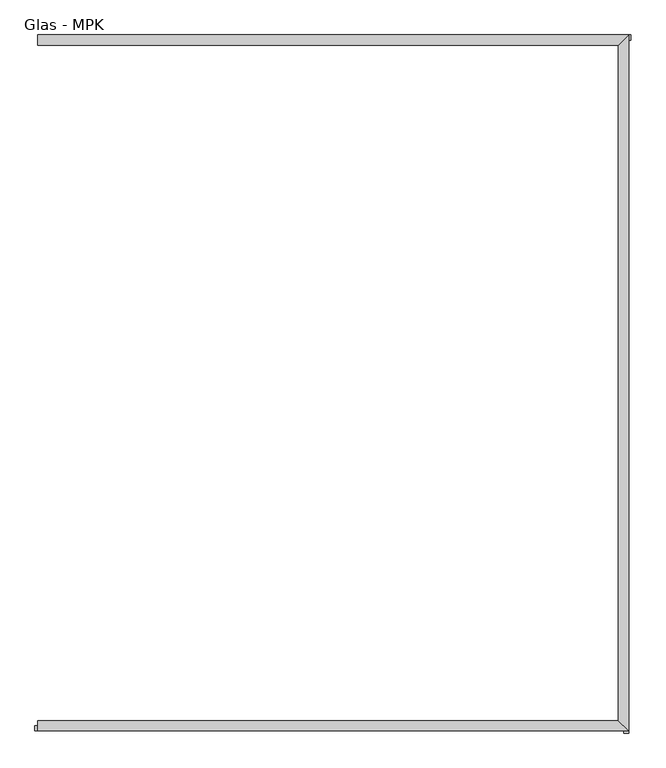
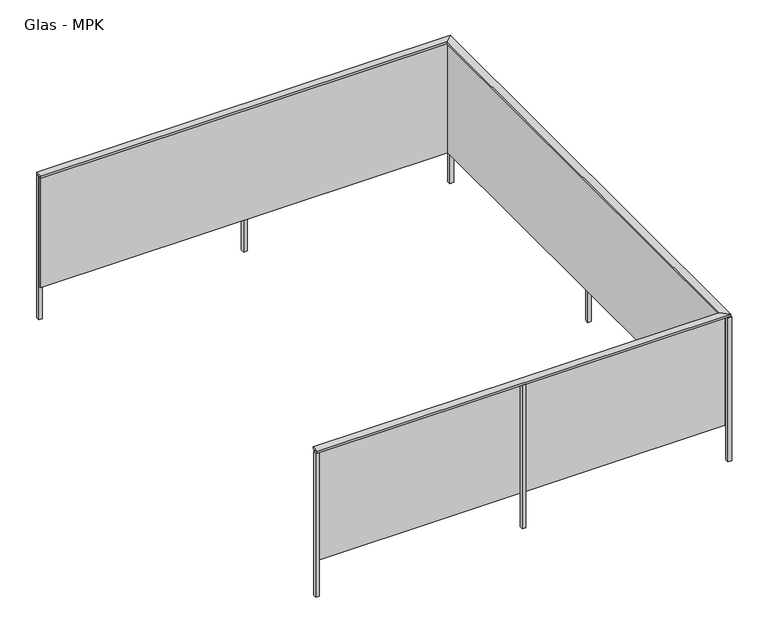
"""IFC4 building model written with IfcOpenShell, lengths in millimetres: railing geometry, Glas - MPK."""

import ifcopenshell
import ifcopenshell.guid

model = None  # the IFC model being written
_history = None  # IfcOwnerHistory: only IFC2X3 demands one
_inside = {}  # id of a spatial element -> (the spatial element, [elements in it])
_under = {}  # id of a project, library or spatial element -> (it, [spatial elements below it])
_declared = {}  # id of a project -> (the project, [libraries it declares])
_typed = {}  # id of a type object -> (the type object, [elements of that type])
_made_of = {}  # id of a material, layer set ... -> (it, [elements and type objects made of it])


def new_model(schema):
    """Start an empty IFC model of exactly this schema.

    Asked for "IFC4X3", IfcOpenShell would pick the latest addendum, in which some entities
    have other attributes; the version numbers below select the first issue.
    IFC2X3 requires an IfcOwnerHistory on every rooted entity: one is made here for all.
    """
    global model, _history
    if schema == "IFC4X3":
        model = ifcopenshell.file(schema_version=(4, 3, 0, 0))
    else:
        model = ifcopenshell.file(schema=schema)
    _inside.clear()
    _under.clear()
    _declared.clear()
    _typed.clear()
    _made_of.clear()
    _history = None
    if model.schema == "IFC2X3":
        org = make("IfcOrganization", Name="unknown")
        user = make(
            "IfcPersonAndOrganization",
            ThePerson=make("IfcPerson", FamilyName="unknown"),
            TheOrganization=org,
        )
        app = make(
            "IfcApplication",
            ApplicationDeveloper=org,
            Version="unknown",
            ApplicationFullName="unknown",
            ApplicationIdentifier="unknown",
        )
        _history = make(
            "IfcOwnerHistory",
            OwningUser=user,
            OwningApplication=app,
            ChangeAction="ADDED",
            CreationDate=0,
        )
    return model


def make(cls, **values):
    """One entity of the class cls with the attributes given. An attribute that is None is left unset."""
    return model.create_entity(
        cls, **{name: value for name, value in values.items() if value is not None}
    )


def rooted(cls, **values):
    """An entity with a GlobalId (a new one), such as an element, a storey or a relation."""
    return make(cls, GlobalId=ifcopenshell.guid.new(), OwnerHistory=_history, **values)


def si_unit(unit_type, name, prefix=None):
    """IfcSIUnit, for example si_unit("LENGTHUNIT", "METRE", prefix="MILLI")."""
    return make("IfcSIUnit", UnitType=unit_type, Prefix=prefix, Name=name)


def assignment(units):
    """IfcUnitAssignment: the units of a project."""
    return None if units is None else make("IfcUnitAssignment", Units=units)


def point(xyz):
    """IfcCartesianPoint."""
    return None if xyz is None else make("IfcCartesianPoint", Coordinates=xyz)


def direction(xyz):
    """IfcDirection."""
    return None if xyz is None else make("IfcDirection", DirectionRatios=xyz)


def frame(location, z_axis=None, x_axis=None):
    """IfcAxis2Placement3D, a coordinate frame: its origin and axes. An axis left out is left unset."""
    return make(
        "IfcAxis2Placement3D",
        Location=point(location),
        Axis=direction(z_axis),
        RefDirection=direction(x_axis),
    )


def origin():
    """The frame at (0, 0, 0) with its axes left unset."""
    return frame((0.0, 0.0, 0.0))


def place(relative_to, where):
    """IfcLocalPlacement: puts the frame where relative to a parent placement (None: the world)."""
    return make(
        "IfcLocalPlacement", PlacementRelTo=relative_to, RelativePlacement=where
    )


def context(
    kind, dimensions, precision=None, world=None, true_north=None, identifier=None
):
    """IfcGeometricRepresentationContext, for example the 3D "Model" context."""
    return make(
        "IfcGeometricRepresentationContext",
        ContextIdentifier=identifier,
        ContextType=kind,
        CoordinateSpaceDimension=dimensions,
        Precision=precision,
        WorldCoordinateSystem=world,
        TrueNorth=true_north,
    )


def project(units=None, contexts=None):
    """IfcProject with its units and contexts."""
    return rooted(
        "IfcProject",
        Name="project",
        RepresentationContexts=contexts,
        UnitsInContext=assignment(units),
    )


def spatial(cls, under=None, at=None, **own):
    """A site, building, storey or space (cls), placed at a placement, below another one or the project."""
    s = rooted(cls, ObjectPlacement=at, **own)
    if under is not None:
        _under.setdefault(under.id(), (under, []))[1].append(s)
    return s


def polyline(points):
    """IfcPolyline through the points."""
    return make("IfcPolyline", Points=[point(p) for p in points])


def outline(outer, holes=None, kind="AREA"):
    """IfcArbitraryClosedProfileDef: a profile drawn as a closed curve; with holes, ...WithVoids."""
    if holes is None:
        return make("IfcArbitraryClosedProfileDef", ProfileType=kind, OuterCurve=outer)
    return make(
        "IfcArbitraryProfileDefWithVoids",
        ProfileType=kind,
        OuterCurve=outer,
        InnerCurves=holes,
    )


def extrude(swept, where, along, depth):
    """IfcExtrudedAreaSolid: the profile swept, set in the frame where, extruded along a direction by depth."""
    return make(
        "IfcExtrudedAreaSolid",
        SweptArea=swept,
        Position=where,
        ExtrudedDirection=direction(along),
        Depth=depth,
    )


def faces_of(points, faces, orient=None, outer=None):
    """IfcFace entities. A face is a list of loops; a loop is a list of indices into points, from 0.

    orient and outer hold one flag for each loop. By default every Orientation is true, the
    first loop of a face is its IfcFaceOuterBound and the others are IfcFaceBound.
    """
    made = []
    for i, loops in enumerate(faces):
        bounds = []
        for j, loop in enumerate(loops):
            is_outer = j == 0 if outer is None else outer[i][j]
            bounds.append(
                make(
                    "IfcFaceOuterBound" if is_outer else "IfcFaceBound",
                    Bound=make("IfcPolyLoop", Polygon=[points[k] for k in loop]),
                    Orientation=True if orient is None else orient[i][j],
                )
            )
        made.append(make("IfcFace", Bounds=bounds))
    return made


def faceted_brep(points, faces, orient=None, outer=None, voids=None):
    """IfcFacetedBrep: a solid bounded by flat faces; with voids (closed shells), ...WithVoids."""
    shared = [point(p) for p in points]
    hull = make("IfcClosedShell", CfsFaces=faces_of(shared, faces, orient, outer))
    if voids is None:
        return make("IfcFacetedBrep", Outer=hull)
    return make(
        "IfcFacetedBrepWithVoids",
        Outer=hull,
        Voids=[
            make(cls, CfsFaces=faces_of(shared, fs, o, b)) for cls, fs, o, b in voids
        ],
    )


def shape(context_of_items, identifier, shape_type, items):
    """IfcShapeRepresentation: the items that make up one representation, for example the "Body"."""
    return make(
        "IfcShapeRepresentation",
        ContextOfItems=context_of_items,
        RepresentationIdentifier=identifier,
        RepresentationType=shape_type,
        Items=items,
    )


def source(mapping_origin, context_of_items, identifier, shape_type, items):
    """IfcRepresentationMap: a shape defined once, which mapped items show again and again."""
    return make(
        "IfcRepresentationMap",
        MappingOrigin=mapping_origin,
        MappedRepresentation=shape(context_of_items, identifier, shape_type, items),
    )


def transform(
    local_origin,
    x_axis=None,
    y_axis=None,
    z_axis=None,
    scale=None,
    scale2=None,
    scale3=None,
    uniform=True,
):
    """IfcCartesianTransformationOperator3D, or its non-uniform kind. x_axis, y_axis, z_axis: its Axis1, 2, 3."""
    if uniform:
        return make(
            "IfcCartesianTransformationOperator3D",
            Axis1=direction(x_axis),
            Axis2=direction(y_axis),
            LocalOrigin=point(local_origin),
            Scale=scale,
            Axis3=direction(z_axis),
        )
    return make(
        "IfcCartesianTransformationOperator3DnonUniform",
        Axis1=direction(x_axis),
        Axis2=direction(y_axis),
        LocalOrigin=point(local_origin),
        Scale=scale,
        Axis3=direction(z_axis),
        Scale2=scale2,
        Scale3=scale3,
    )


def mapped(mapping_source, mapping_target):
    """IfcMappedItem: shows the shape of a source again, moved by a transform."""
    return make(
        "IfcMappedItem", MappingSource=mapping_source, MappingTarget=mapping_target
    )


def made_of(thing, what):
    """Note that an element or type object is made of a material, layer set ...; save() writes the relation."""
    if what is not None:
        _made_of.setdefault(what.id(), (what, []))[1].append(thing)
    return thing


def element(
    cls,
    number,
    at=None,
    inside=None,
    cuts=None,
    type_object=None,
    material=None,
    context=None,
    identifier="Body",
    shape_type=None,
    held_by="IfcProductDefinitionShape",
    body=None,
    shapes=None,
    **own,
):
    """One element of the class cls, such as IfcWall. Its Tag is "e" and its number.

    at: its placement. inside: the storey or other place that contains it. cuts: it is an
    opening in that element (IfcRelVoidsElement). A single representation is given by context,
    identifier, shape_type and body (its items); several are given by shapes. held_by: the class
    of the entity that holds the representations. save() writes the other relations.
    """
    e = rooted(cls, Tag="e%d" % number, ObjectPlacement=at, **own)
    if body is not None:
        shapes = [shape(context, identifier, shape_type, body)]
    if shapes is not None:
        e.Representation = make(held_by, Representations=shapes)
    if inside is not None:
        _inside.setdefault(inside.id(), (inside, []))[1].append(e)
    if cuts is not None:
        rooted(
            "IfcRelVoidsElement", RelatingBuildingElement=cuts, RelatedOpeningElement=e
        )
    if type_object is not None:
        _typed.setdefault(type_object.id(), (type_object, []))[1].append(e)
    return made_of(e, material)


def aggregate(whole, parts):
    """IfcRelAggregates: a whole, such as a stair, and the parts it consists of."""
    return rooted("IfcRelAggregates", RelatingObject=whole, RelatedObjects=parts)


def save(model, path):
    """Write the relations noted so far, then the file.

    IfcRelAggregates (storeys below a building ...), IfcRelContainedInSpatialStructure (elements
    in a storey), IfcRelDefinesByType, IfcRelAssociatesMaterial and IfcRelDeclares: one each for
    every whole, place, type object, material and project.
    """
    for whole, parts in _under.values():
        aggregate(whole, parts)
    for where, things in _inside.values():
        rooted(
            "IfcRelContainedInSpatialStructure",
            RelatedElements=things,
            RelatingStructure=where,
        )
    for kind, things in _typed.values():
        rooted("IfcRelDefinesByType", RelatedObjects=things, RelatingType=kind)
    for what, things in _made_of.values():
        rooted("IfcRelAssociatesMaterial", RelatedObjects=things, RelatingMaterial=what)
    for by, libraries in _declared.values():
        rooted("IfcRelDeclares", RelatingContext=by, RelatedDefinitions=libraries)
    model.write(path)


def glas_mpk_050cb379(model_context):
    return source(origin(), model_context, "Body", "SolidModel", [
        faceted_brep([(28820.3199184, 1288.5335867, 3843.2628643), (28820.3199184, 1238.5335867, 3843.2628643), (28820.3199184, 1238.5335867, 3856.7371357), (28820.3199184, 1288.5335867, 3856.7371357), (31660.3199184, 1288.5335867, 3843.2628643), (31610.3199184, 1238.5335867, 3843.2628643), (31610.3199184, 1238.5335867, 3856.7371357), (31660.3199184, 1288.5335867, 3856.7371357), (31660.3199184, -2052.1957594, 3843.2628643), (31610.3199184, -2002.1957594, 3843.2628643), (31610.3199184, -2002.1957594, 3856.7371357), (31660.3199184, -2052.1957594, 3856.7371357), (28820.3199184, -2052.1957594, 3843.2628643), (28820.3199184, -2052.1957594, 3856.7371357), (28820.3199184, -2002.1957594, 3856.7371357), (28820.3199184, -2002.1957594, 3843.2628643)], [[[0, 1, 2, 3]], [[1, 0, 4, 5]], [[2, 1, 5, 6]], [[3, 2, 6, 7]], [[0, 3, 7, 4]], [[5, 4, 8, 9]], [[6, 5, 9, 10]], [[7, 6, 10, 11]], [[4, 7, 11, 8]], [[12, 13, 14, 15]], [[9, 8, 12, 15]], [[10, 9, 15, 14]], [[11, 10, 14, 13]], [[8, 11, 13, 12]]]),
        faceted_brep([(28820.3199184, 1248.5335867, 3842.8769824), (28820.3199184, 1262.7257107, 3842.8769824), (28820.3199184, 1262.7257107, 3042.8769824), (28820.3199184, 1248.5335867, 3042.8769824), (31620.3199184, 1248.5335867, 3842.8769824), (31634.5120424, 1262.7257107, 3842.8769824), (31634.5120424, 1262.7257107, 3042.8769824), (31620.3199184, 1248.5335867, 3042.8769824), (31620.3199184, -2012.1957594, 3842.8769824), (31634.5120424, -2026.3878834, 3842.8769824), (31634.5120424, -2026.3878834, 3042.8769824), (31620.3199184, -2012.1957594, 3042.8769824), (28820.3199184, -2012.1957594, 3842.8769824), (28820.3199184, -2012.1957594, 3042.8769824), (28820.3199184, -2026.3878834, 3042.8769824), (28820.3199184, -2026.3878834, 3842.8769824)], [[[0, 1, 2, 3]], [[1, 0, 4, 5]], [[2, 1, 5, 6]], [[3, 2, 6, 7]], [[0, 3, 7, 4]], [[5, 4, 8, 9]], [[6, 5, 9, 10]], [[7, 6, 10, 11]], [[4, 7, 11, 8]], [[12, 13, 14, 15]], [[9, 8, 12, 15]], [[10, 9, 15, 14]], [[11, 10, 14, 13]], [[8, 11, 13, 12]]]),
        extrude(outline(polyline([(30251.5699184, -2027.1957594), (30251.5699184, -2052.1957594), (30226.5699184, -2052.1957594), (30226.5699184, -2027.1957594), (30251.5699184, -2027.1957594)])), frame((0.0, 0.0, 2800.0), z_axis=(0.0, 0.0, 1.0), x_axis=(1.0, 0.0, 0.0)), (0.0, 0.0, 1.0), 1043.2628643),
        extrude(outline(polyline([(31635.3199184, -369.3310864), (31660.3199184, -369.3310864), (31660.3199184, -394.3310864), (31635.3199184, -394.3310864), (31635.3199184, -369.3310864)])), frame((0.0, 0.0, 2800.0), z_axis=(0.0, 0.0, 1.0), x_axis=(1.0, 0.0, 0.0)), (0.0, 0.0, 1.0), 1043.2628643),
        extrude(outline(polyline([(30226.5699184, 1263.5335867), (30226.5699184, 1288.5335867), (30251.5699184, 1288.5335867), (30251.5699184, 1263.5335867), (30226.5699184, 1263.5335867)])), frame((0.0, 0.0, 2800.0), z_axis=(0.0, 0.0, 1.0), x_axis=(1.0, 0.0, 0.0)), (0.0, 0.0, 1.0), 1043.2628643),
        extrude(outline(polyline([(31635.3199184, -2037.1957594), (31660.3199184, -2037.1957594), (31660.3199184, -2062.1957594), (31635.3199184, -2062.1957594), (31635.3199184, -2037.1957594)])), frame((0.0, 0.0, 2800.0), z_axis=(0.0, 0.0, 1.0), x_axis=(1.0, 0.0, 0.0)), (0.0, 0.0, 1.0), 1043.2628643),
        extrude(outline(polyline([(31645.3199184, 1263.5335867), (31645.3199184, 1288.5335867), (31670.3199184, 1288.5335867), (31670.3199184, 1263.5335867), (31645.3199184, 1263.5335867)])), frame((0.0, 0.0, 2800.0), z_axis=(0.0, 0.0, 1.0), x_axis=(1.0, 0.0, 0.0)), (0.0, 0.0, 1.0), 1043.2628643),
        extrude(outline(polyline([(28832.8199184, -2027.1957594), (28832.8199184, -2052.1957594), (28807.8199184, -2052.1957594), (28807.8199184, -2027.1957594), (28832.8199184, -2027.1957594)])), frame((0.0, 0.0, 2800.0), z_axis=(0.0, 0.0, 1.0), x_axis=(1.0, 0.0, 0.0)), (0.0, 0.0, 1.0), 1043.2628643),
        extrude(outline(polyline([(28820.3199184, 1263.5335867), (28820.3199184, 1288.5335867), (28845.3199184, 1288.5335867), (28845.3199184, 1263.5335867), (28820.3199184, 1263.5335867)])), frame((0.0, 0.0, 2800.0), z_axis=(0.0, 0.0, 1.0), x_axis=(1.0, 0.0, 0.0)), (0.0, 0.0, 1.0), 1043.2628643),
    ])


if __name__ == "__main__":
    model = new_model("IFC4")
    model_context = context("Model", 3, world=origin())
    ifc_project = project(units=[si_unit("LENGTHUNIT", "METRE", prefix="MILLI")], contexts=[model_context])
    site = spatial("IfcSite", under=ifc_project)
    building = spatial("IfcBuilding", under=site)
    placement = place(None, origin())
    glas_mpk_shape = glas_mpk_050cb379(model_context)
    element("IfcRailing", 1, ObjectType="Glas - MPK", at=placement, inside=building, context=model_context, shape_type="MappedRepresentation", body=[
        mapped(glas_mpk_shape, transform((0.0, 0.0, 0.0), x_axis=(1.0, 0.0, 0.0), y_axis=(0.0, 1.0, 0.0), z_axis=(0.0, 0.0, 1.0))),
    ])
    save(model, "model.ifc")

# Revit data of these elements
# Element 1 (IfcRailing, "Glas - MPK")
#   Materials on its faces: "Metal - Aluminum", "Window - Glass"
# Materials
#   "Metal - Aluminum": class "Unassigned", colour RGB 247 247 247, transparency 0, Comments = "Rendering appearance not upgraded "
#   "Window - Glass": class "Glas", colour RGB 128 128 255, transparency 0.75
